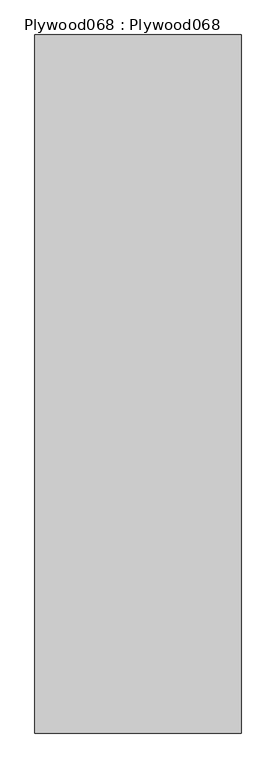
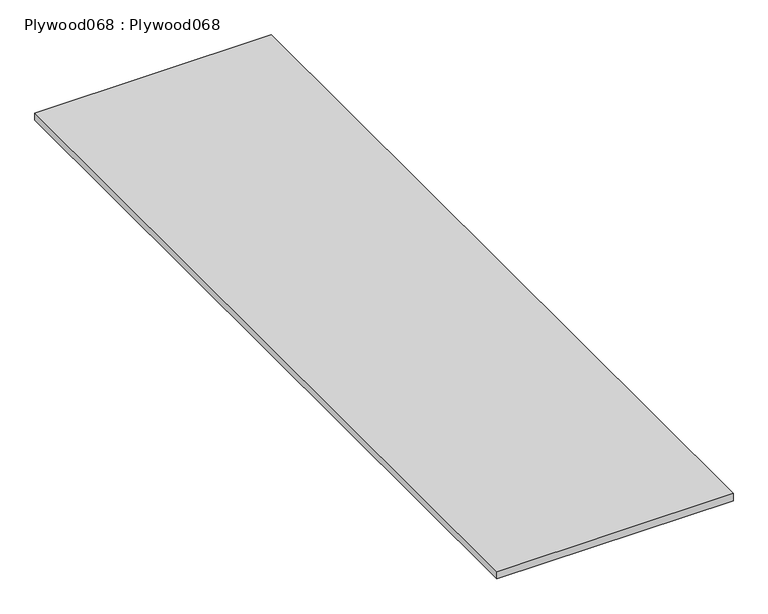
"""IFC4 building model written with IfcOpenShell, lengths in millimetres: proxy geometry, Plywood068 : Plywood068."""

from ifc_helpers import new_model, si_unit, frame, origin, place, context, project, spatial, polyline, outline, extrude, source, transform, mapped, element, save


def plywood068_plywood068_7b2ffb50(model_context):
    return source(origin(), model_context, "Body", "SweptSolid", [
        extrude(outline(polyline([(-9298.3737014, 7982.1531721), (-9888.9237014, 7982.1531721), (-9888.9237014, 9982.1531721), (-9298.3737014, 9982.1531721), (-9298.3737014, 7982.1531721)])), frame((0.0, 0.0, 39934.8960083), z_axis=(0.0, 0.0, 1.0), x_axis=(1.0, 0.0, 0.0)), (0.0, 0.0, 1.0), 19.05),
    ])


if __name__ == "__main__":
    model = new_model("IFC4")
    model_context = context("Model", 3, world=origin())
    ifc_project = project(units=[si_unit("LENGTHUNIT", "METRE", prefix="MILLI")], contexts=[model_context])
    site = spatial("IfcSite", under=ifc_project)
    building = spatial("IfcBuilding", under=site)
    placement = place(None, origin())
    plywood068_plywood068_shape = plywood068_plywood068_7b2ffb50(model_context)
    element("IfcBuildingElementProxy", 1, Name="Plywood068 : Plywood068", ObjectType="Plywood068 : Plywood068", at=placement, inside=building, context=model_context, shape_type="MappedRepresentation", body=[
        mapped(plywood068_plywood068_shape, transform((0.0, 0.0, 0.0), x_axis=(1.0, 0.0, 0.0), y_axis=(0.0, 1.0, 0.0), z_axis=(0.0, 0.0, 1.0))),
    ])
    save(model, "model.ifc")

# Revit data of these elements
# Type "Plywood068 : Plywood068"
#   NameOverride = "Plywood068"
# Element 1 (IfcBuildingElementProxy, "Plywood068 : Plywood068")
#   Materials on its faces: "CDX PLYWOOD - SEE STRUCTURAL DWGS"
# Materials
#   "CDX PLYWOOD - SEE STRUCTURAL DWGS": class "Unassigned", colour RGB 177 130 114, transparency 0, Cost = 0
